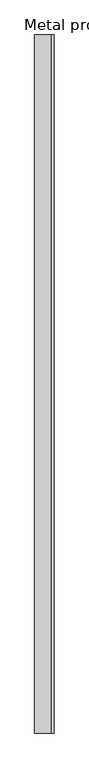
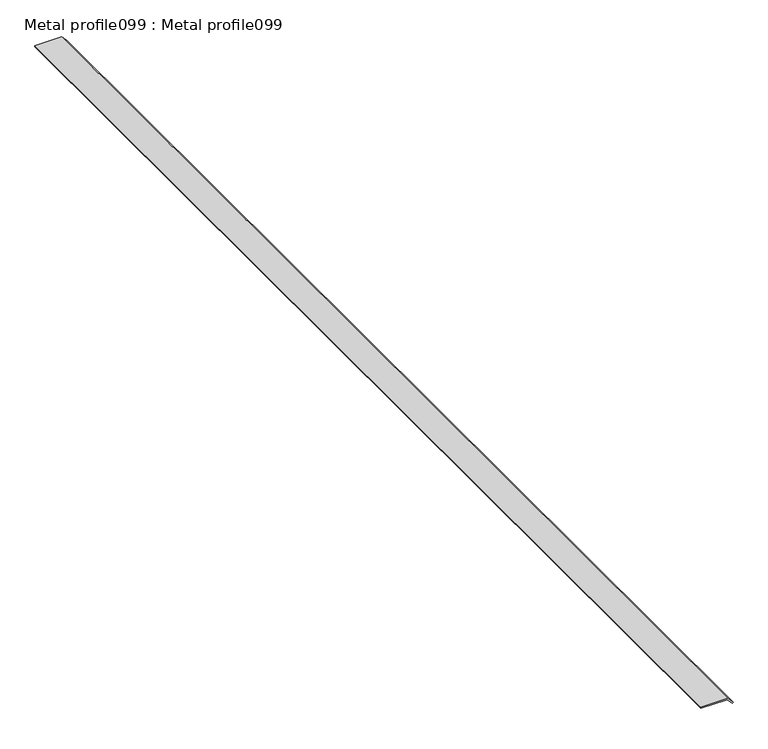
"""IFC4 building model written with IfcOpenShell, lengths in millimetres: proxy geometry, Metal profile099 : Metal profile099."""

from ifc_helpers import new_model, si_unit, frame, origin, place, context, project, spatial, polyline, outline, extrude, source, transform, mapped, element, save


def metal_profile099_metal_profile099_c8f02b68(model_context):
    return source(origin(), model_context, "Body", "SweptSolid", [
        extrude(outline(polyline([(43002.0078125, 16606.9570313), (43002.0078125, 16652.1835459), (42991.9066174, 16661.2456667), (42993.2421875, 16662.734375), (43004.0078125, 16653.0761719), (43004.0078125, 16606.9570313), (43002.0078125, 16606.9570313)])), frame((0.0, 7982.1435747, 0.0), z_axis=(0.0, 1.0, 0.0), x_axis=(0.0, 0.0, 1.0)), (0.0, 0.0, 1.0), 2000.0),
    ])


if __name__ == "__main__":
    model = new_model("IFC4")
    model_context = context("Model", 3, world=origin())
    ifc_project = project(units=[si_unit("LENGTHUNIT", "METRE", prefix="MILLI")], contexts=[model_context])
    site = spatial("IfcSite", under=ifc_project)
    building = spatial("IfcBuilding", under=site)
    placement = place(None, origin())
    metal_profile099_metal_profile099_shape = metal_profile099_metal_profile099_c8f02b68(model_context)
    element("IfcBuildingElementProxy", 1, Name="Metal profile099 : Metal profile099", ObjectType="Metal profile099 : Metal profile099", at=placement, inside=building, context=model_context, shape_type="MappedRepresentation", body=[
        mapped(metal_profile099_metal_profile099_shape, transform((0.0, 0.0, 0.0), x_axis=(1.0, 0.0, 0.0), y_axis=(0.0, 1.0, 0.0), z_axis=(0.0, 0.0, 1.0))),
    ])
    save(model, "model.ifc")

# Revit data of these elements
# Type "Metal profile099 : Metal profile099"
#   NameOverride = "Metal profile099"
# Element 1 (IfcBuildingElementProxy, "Metal profile099 : Metal profile099")
#   Materials on its faces: "ANGLE TRIM 1419"
# Materials
#   "ANGLE TRIM 1419": class "Unassigned", colour RGB 250 255 0, transparency 0
